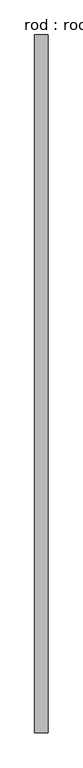
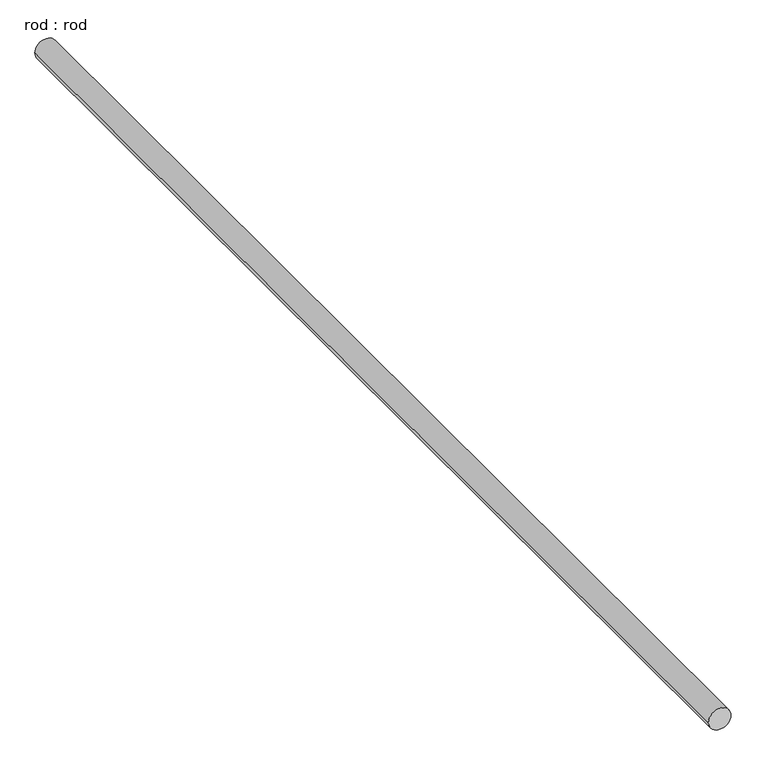
"""IFC4 building model written with IfcOpenShell, lengths in millimetres: proxy geometry, rod : rod."""

from ifc_helpers import new_model, si_unit, point, frame, frame_2d, origin, place, context, project, spatial, circle_curve, trimmed, segment, composite_curve, outline, extrude, source, transform, mapped, element, save


def rod_rod_93724543(model_context):
    return source(origin(), model_context, "Body", "SweptSolid", [
        extrude(outline(composite_curve([segment(trimmed(circle_curve(frame_2d((0.0108462, 0.0)), 200.0), [point((0.0108462, 200.0))], [point((0.0108462, -200.0))], False, "CARTESIAN"), True, "CONTINUOUS"), segment(trimmed(circle_curve(frame_2d((0.0108462, 0.0)), 200.0), [point((0.0108462, -200.0))], [point((0.0108462, 200.0))], False, "CARTESIAN"), True, "CONTINUOUS")], self_intersect=False)), frame((0.0, -6359.3080017, 0.0), z_axis=(0.0, 1.0, 0.0), x_axis=(0.0, 0.0, 1.0)), (0.0, 0.0, 1.0), 20904.0732341),
    ])


if __name__ == "__main__":
    model = new_model("IFC4")
    model_context = context("Model", 3, world=origin())
    ifc_project = project(units=[si_unit("LENGTHUNIT", "METRE", prefix="MILLI")], contexts=[model_context])
    site = spatial("IfcSite", under=ifc_project)
    building = spatial("IfcBuilding", under=site)
    placement = place(None, origin())
    rod_rod_shape = rod_rod_93724543(model_context)
    element("IfcBuildingElementProxy", 1, Name="rod : rod", ObjectType="rod : rod", at=placement, inside=building, context=model_context, shape_type="MappedRepresentation", body=[
        mapped(rod_rod_shape, transform((0.0, 0.0, 0.0), x_axis=(1.0, 0.0, 0.0), y_axis=(0.0, 1.0, 0.0), z_axis=(0.0, 0.0, 1.0))),
    ])
    save(model, "model.ifc")

# Revit data of these elements
# Type "rod : rod"
#   Default Elevation = 0
